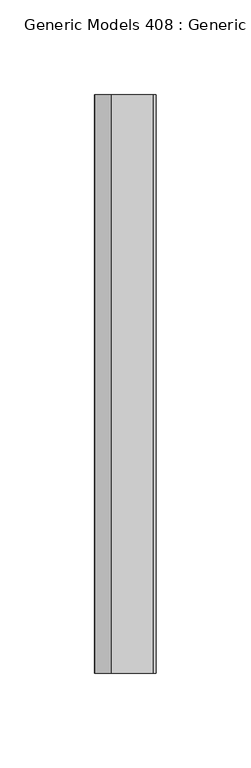
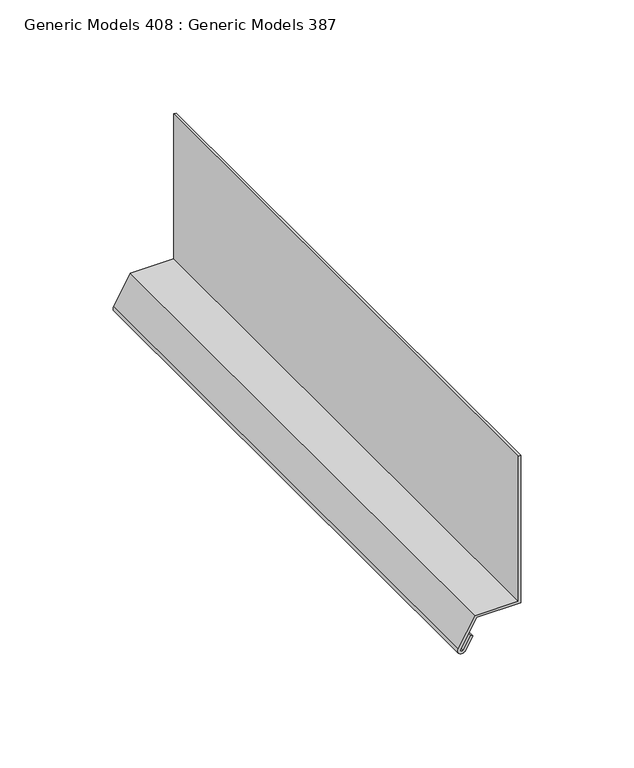
"""IFC4 building model written with IfcOpenShell, lengths in millimetres: proxy geometry, Generic Models 408 : Generic Models 387."""

from ifc_helpers import new_model, si_unit, point, frame, frame_2d, origin, place, context, project, spatial, polyline, circle_curve, trimmed, segment, composite_curve, outline, extrude, source, transform, mapped, element, save


def generic_models_408_generic_models_387_da4452d0(model_context):
    return source(origin(), model_context, "Body", "SweptSolid", [
        extrude(outline(composite_curve([segment(polyline([(129105.9531523, -7051.7971429), (129105.9531523, -7053.0869866), (129027.6785371, -7053.0869866), (129027.6785371, -7075.2031846), (129012.7559245, -7083.818759)]), True, "CONTINUOUS"), segment(trimmed(circle_curve(frame_2d((129011.6669278, -7081.9325614)), 2.1779933), [point((129012.7559245, -7083.818759))], [point((129010.5779312, -7080.0463638))], False, "CARTESIAN"), True, "CONTINUOUS"), segment(polyline([(129010.5779312, -7080.0463638), (129017.0690189, -7076.2987326), (129017.7139408, -7077.41577), (129011.0758475, -7081.248275)]), True, "CONTINUOUS"), segment(trimmed(circle_curve(frame_2d((129011.6524708, -7081.9409082)), 0.9012409), [point((129011.0758475, -7081.248275))], [point((129011.6550969, -7082.8421453))], True, "CARTESIAN"), True, "CONTINUOUS"), segment(polyline([(129011.6550969, -7082.8421453), (129026.3886933, -7074.3356994), (129026.3886933, -7051.7971429), (129105.9531523, -7051.7971429)]), True, "CONTINUOUS")], self_intersect=False)), frame((0.0, -4250.542257, 0.0), z_axis=(0.0, 1.0, 0.0), x_axis=(0.0, 0.0, 1.0)), (0.0, 0.0, 1.0), 304.8),
    ])


if __name__ == "__main__":
    model = new_model("IFC4")
    model_context = context("Model", 3, world=origin())
    ifc_project = project(units=[si_unit("LENGTHUNIT", "METRE", prefix="MILLI")], contexts=[model_context])
    site = spatial("IfcSite", under=ifc_project)
    building = spatial("IfcBuilding", under=site)
    placement = place(None, origin())
    generic_models_408_generic_models_387_shape = generic_models_408_generic_models_387_da4452d0(model_context)
    element("IfcBuildingElementProxy", 1, Name="Generic Models 408 : Generic Models 387", ObjectType="Generic Models 408 : Generic Models 387", at=placement, inside=building, context=model_context, shape_type="MappedRepresentation", body=[
        mapped(generic_models_408_generic_models_387_shape, transform((0.0, 0.0, 0.0), x_axis=(1.0, 0.0, 0.0), y_axis=(0.0, 1.0, 0.0), z_axis=(0.0, 0.0, 1.0))),
    ])
    save(model, "model.ifc")

# Revit data of these elements
# Element 1 (IfcBuildingElementProxy, "Generic Models 408 : Generic Models 387")
#   Materials on its faces: "_CONT. 16 GA. COPPER DRIP FLASHING"
# Materials
#   "_CONT. 16 GA. COPPER DRIP FLASHING": class "Metal", colour RGB 199 199 199, transparency 0, Description = "Structural steel 50ksi", Cost = 0
